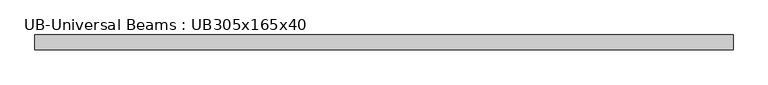
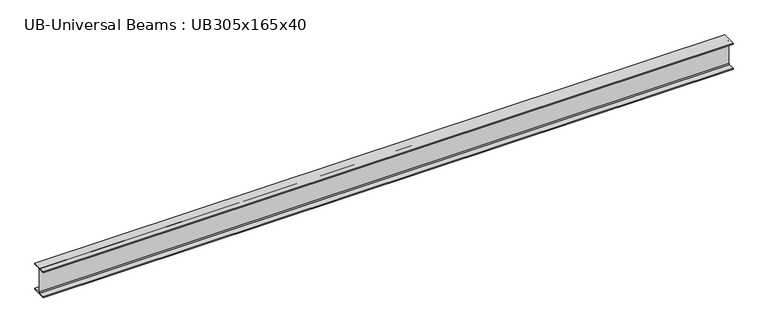
"""IFC4 building model written with IfcOpenShell, lengths in millimetres: beam geometry, UB-Universal Beams : UB305x165x40."""

from ifc_helpers import new_model, si_unit, point, frame, frame_2d, origin, place, context, project, spatial, polyline, circle_curve, trimmed, segment, composite_curve, outline, extrude, source, transform, mapped, element, save


def ub_universal_beams_ub305x165x40_37dc1813(model_context):
    return source(origin(), model_context, "Body", "SweptSolid", [
        extrude(outline(composite_curve([segment(polyline([(82.5, -141.5), (82.5, -151.7), (-82.5, -151.7), (-82.5, -141.5), (-11.9, -141.5)]), True, "CONTINUOUS"), segment(trimmed(circle_curve(frame_2d((-11.9, -132.6)), 8.9), [point((-11.9, -141.5))], [point((-3.0, -132.6))], True, "CARTESIAN"), True, "CONTINUOUS"), segment(polyline([(-3.0, -132.6), (-3.0, 132.6)]), True, "CONTINUOUS"), segment(trimmed(circle_curve(frame_2d((-11.9, 132.6)), 8.9), [point((-3.0, 132.6))], [point((-11.9, 141.5))], True, "CARTESIAN"), True, "CONTINUOUS"), segment(polyline([(-11.9, 141.5), (-82.5, 141.5), (-82.5, 151.7), (82.5, 151.7), (82.5, 141.5), (11.9, 141.5)]), True, "CONTINUOUS"), segment(trimmed(circle_curve(frame_2d((11.9, 132.6)), 8.9), [point((11.9, 141.5))], [point((3.0, 132.6))], True, "CARTESIAN"), True, "CONTINUOUS"), segment(polyline([(3.0, 132.6), (3.0, -132.6)]), True, "CONTINUOUS"), segment(trimmed(circle_curve(frame_2d((11.9, -132.6)), 8.9), [point((3.0, -132.6))], [point((11.9, -141.5))], True, "CARTESIAN"), True, "CONTINUOUS"), segment(polyline([(11.9, -141.5), (82.5, -141.5)]), True, "CONTINUOUS")], self_intersect=False)), frame((-3834.6, 0.0, 0.0), z_axis=(1.0, 0.0, 0.0), x_axis=(0.0, 1.0, 0.0)), (0.0, 0.0, 1.0), 7669.2),
    ])


if __name__ == "__main__":
    model = new_model("IFC4")
    model_context = context("Model", 3, world=origin())
    ifc_project = project(units=[si_unit("LENGTHUNIT", "METRE", prefix="MILLI")], contexts=[model_context])
    site = spatial("IfcSite", under=ifc_project)
    building = spatial("IfcBuilding", under=site)
    placement = place(None, origin())
    ub_universal_beams_ub305x165x40_shape = ub_universal_beams_ub305x165x40_37dc1813(model_context)
    element("IfcBeam", 1, ObjectType="UB-Universal Beams : UB305x165x40", at=placement, inside=building, context=model_context, shape_type="MappedRepresentation", body=[
        mapped(ub_universal_beams_ub305x165x40_shape, transform((0.0, 0.0, 0.0), x_axis=(1.0, 0.0, 0.0), y_axis=(0.0, 1.0, 0.0), z_axis=(0.0, 0.0, 1.0))),
    ])
    save(model, "model.ifc")

# Revit data of these elements
# Type "UB-Universal Beams : UB305x165x40"
#   Section Name Key = "UB305X165X40"
#   Width = 16.5 cm
#   Web Thickness = 0.6 cm
#   Web Fillet = 0.89 cm
#   Warping Constant = 164000.0 cm⁶
#   Torsional Moment of Inertia = 14.70 cm⁴
#   Section Area = 51.3 cm²
#   Plastic Modulus weak axis = 142.0 cm³
#   Plastic Modulus strong axis = 623.0 cm³
#   Nominal Weight = 40.2999 kgf/m
#   Moment of Inertia weak axis = 764.00 cm⁴
#   Moment of Inertia strong axis = 8503.00 cm⁴
#   Height = 30.34 cm
#   Flange Thickness = 1.02 cm
#   Elastic Modulus weak axis = 92.6 cm³
#   Elastic Modulus strong axis = 560.0 cm³
#   Centroid Vertical = 15.17 cm
#   Centroid Horizontal = 8.25 cm
#   Bolt Spacing = 9.0 cm
#   Length [instance default] = 1500 mm
#   Structural Material [instance default] = Metal - Steel 43-275
#   Type Comments = ""
#   Assembly Code = ""
# Element 1 (IfcBeam, "UB-Universal Beams : UB305x165x40")
#   Materials on its faces: "Metal - Steel 43-275"
# Materials
#   "Metal - Steel 43-275": class "Metal", colour RGB 247 247 247, transparency 0, Cost = 0
